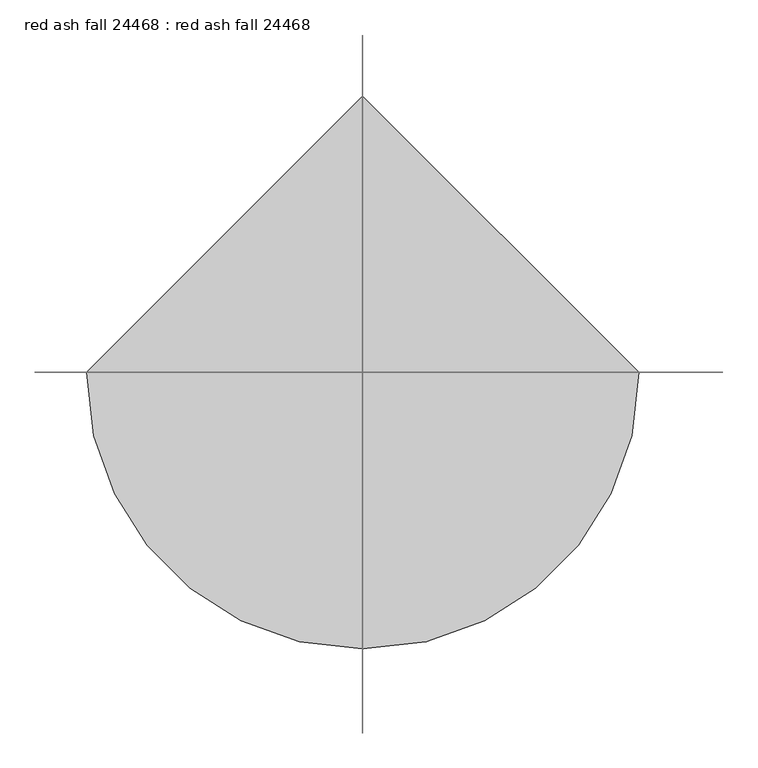
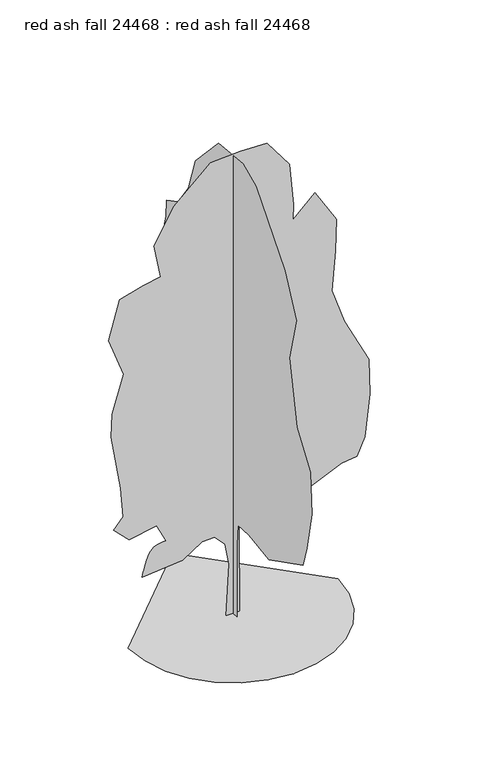
"""IFC4 building model written with IfcOpenShell, lengths in millimetres: proxy geometry, red ash fall 24468 : red ash fall 24468."""

from ifc_helpers import new_model, si_unit, origin, place, context, project, spatial, triangles, source, transform, mapped, element, save


def red_ash_fall_24468_red_ash_fall_24468_841d54ac(model_context):
    return source(origin(), model_context, "Body", "Tessellation", [
        triangles([(-1644.9506115, 0.0, 6.19e-05), (-1601.463295, -376.9127495, 6.19e-05), (-1477.6130058, -723.0483805, 6.19e-05), (-1283.3159992, -1028.488167, 6.19e-05), (-1028.488167, -1283.3159992, 6.19e-05), (-723.0483805, -1477.6130058, 6.19e-05), (-376.9127495, -1601.463295, 6.19e-05), (7.19e-05, -1644.9506115, 6.19e-05), (376.9127495, -1601.463295, 6.19e-05), (723.0483805, -1477.6130058, 6.19e-05), (1028.488167, -1283.3159992, 6.19e-05), (1283.3159992, -1028.488167, 6.19e-05), (1477.6130058, -723.0483805, 6.19e-05), (1601.463295, -376.9127495, 6.19e-05), (1644.9506115, 0.0001438, 6.19e-05), (-0.0002157, 1644.9506115, 6.19e-05), (-1.07e-05, -102.8462751, 0.0), (2.5e-05, -101.2465816, 1194.5531759), (3.23e-05, -129.8817524, 1537.8007565), (7e-07, -438.8252131, 1558.1640484), (-5.78e-05, -976.3902569, 1478.3064228), (-0.0001405, -1903.6900509, 1948.6758224), (-0.0001413, -2011.2029652, 2298.0931572), (-0.0001361, -2145.594326, 2943.1712242), (-0.0001119, -2105.2794903, 3615.1275925), (-5.81e-05, -1740.3808331, 4141.0085747), (-5.5e-06, -1527.397031, 5160.6396515), (-3.5e-06, -1715.5422329, 5886.3424484), (4.79e-05, -1406.4448208, 6531.4257477), (0.0001569, -626.9729948, 7458.7278671), (0.0001985, -273.1995851, 7618.189064), (0.0002662, 394.4006355, 7552.8093338), (0.0003121, 1026.0396246, 6880.8276764), (0.0003149, 1214.1899134, 6316.3894547), (0.0003323, 1496.4089516, 5913.2158081), (0.0003598, 1805.5114506, 5751.9512329), (0.0003531, 1818.9506012, 5483.1688019), (0.0003523, 1899.5853596, 5174.076622), (0.0003275, 1765.1941441, 4811.2124336), (0.0003297, 1886.146209, 4461.7849251), (0.0003279, 2007.0984192, 3977.9914902), (0.0003211, 1980.220118, 3843.6002747), (0.0002877, 1751.7549934, 3521.0461258), (0.0002729, 1737.3099449, 3077.5624397), (0.0002632, 1724.8766922, 2795.3433289), (0.0002542, 1738.3158428, 2445.9236687), (0.0002412, 1751.7549934, 1962.1149731), (0.0002172, 1563.6071754, 1814.2846069), (0.0001807, 1214.1899134, 1814.2846069), (0.0001827, 1375.4593575, 1317.0369061), (0.0001715, 1348.4948696, 1034.8838522), (0.0001516, 1103.0294746, 1227.8347927), (9.86e-05, 629.4621597, 1106.7073751), (9.8e-05, 551.7102922, 1357.0597538), (6.29e-05, 215.912475, 1354.0015102), (5.03e-05, 130.8009823, 1228.3325821), (3.27e-05, 79.5491688, 818.2830471), (1.17e-05, 112.1657825, 1.28e-05), (-110.8706308, 4.8e-06, 4.46e-05), (-66.7115076, -9.64e-05, 833.5001415), (-129.3072053, -0.000136, 1187.9415882), (-290.7865203, -0.00015, 1365.317244), (-483.63585, -0.0001408, 1358.6954098), (-796.2663677, -0.000103, 1155.7673893), (-1427.9079002, -6.9e-05, 1102.0109322), (-1419.1702068, -7.35e-05, 1136.7631714), (-1409.8433052, -7.82e-05, 1172.6914289), (-1399.343074, -8.32e-05, 1210.9717232), (-1387.0798691, -8.87e-05, 1252.7800724), (-1372.4647728, -9.49e-05, 1299.2874081), (-1354.9133732, -0.0001019, 1351.6722919), (-1333.8339912, -0.0001099, 1411.110815), (-1307.2681709, -0.0001176, 1466.2389908), (-1274.3547729, -0.0001239, 1506.5562973), (-1236.1533257, -0.0001289, 1534.5292992), (-1193.7200872, -0.0001329, 1552.6318279), (-1148.1144407, -0.0001362, 1563.327832), (-1100.3903915, -0.000139, 1569.0885269), (-1051.6097208, -0.0001415, 1572.3803318), (-1199.4401596, -0.0001703, 1868.0410641), (-1629.4947235, -0.0001418, 1787.4063057), (-1871.3989986, -0.0001601, 2029.3105808), (-1723.5686325, -0.0001874, 2204.0192482), (-1763.8834682, -0.0002433, 2687.8251823), (-1911.7164505, -0.0003442, 3588.2545235), (-1898.477869, -0.0003892, 3961.1515297), (-1719.9160938, -0.0004688, 4563.30867), (-1952.033757, -0.0005347, 5200.9494003), (-1777.3226189, -0.000616, 5819.1593399), (-1414.4661335, -0.0006447, 5926.6521973), (-1138.4116173, -0.0006626, 5975.3439926), (-1239.7574661, -0.0007228, 6517.9893585), (-930.6575832, -0.000802, 7068.9906097), (-352.7751603, -0.0008897, 7593.1190826), (117.5945209, -0.0009135, 7619.9924423), (534.2071818, -0.0009301, 7606.5560532), (883.6270237, -0.0008893, 7136.1737183), (947.8711401, -0.00081, 6447.504126), (938.6459038, -0.0007795, 6194.9520996), (1286.8008156, -0.0008333, 6517.9893585), (1622.7789997, -0.0007823, 5966.9875259), (1609.3398491, -0.0007196, 5446.5163879), (1549.4568764, -0.00064, 4800.6459274), (1743.7310646, -0.0005809, 4233.337532), (2131.7614494, -0.0005067, 3469.2048134), (2144.1338047, -0.0004386, 2892.8030777), (2066.2700981, -0.0003531, 2204.0192482), (1945.3180332, -0.0003141, 1921.7976665), (1703.4137581, -0.0003003, 1894.9193653), (1233.0443584, -0.0002542, 1679.8933914), (816.4288725, -0.0002007, 1384.2325138), (257.4769983, -0.0002049, 1624.5671173), (93.0507792, -0.0001766, 1447.6334404), (104.1551341, -4.6e-06, 3.52e-05)], [[15, 16, 1], [14, 15, 1], [14, 1, 2], [13, 14, 2], [13, 2, 3], [13, 3, 4], [12, 13, 4], [11, 12, 4], [11, 4, 5], [11, 5, 6], [11, 6, 7], [11, 7, 8], [11, 8, 9], [11, 9, 10], [50, 51, 52], [57, 58, 17], [57, 17, 18], [56, 57, 18], [56, 18, 19], [55, 56, 19], [49, 50, 52], [52, 53, 54], [49, 52, 54], [35, 36, 37], [46, 47, 48], [46, 48, 49], [21, 22, 23], [20, 21, 23], [20, 23, 24], [20, 24, 25], [20, 25, 26], [19, 20, 26], [19, 26, 27], [45, 46, 49], [31, 32, 33], [30, 31, 33], [29, 30, 33], [29, 33, 34], [28, 29, 34], [27, 28, 34], [19, 27, 34], [19, 34, 35], [19, 35, 37], [19, 37, 38], [19, 38, 39], [19, 39, 40], [19, 40, 41], [19, 41, 42], [19, 42, 43], [19, 43, 44], [19, 44, 45], [19, 45, 49], [19, 49, 54], [55, 19, 54], [64, 65, 66], [64, 66, 67], [64, 67, 68], [99, 100, 101], [64, 68, 69], [64, 69, 70], [64, 70, 71], [114, 59, 60], [113, 114, 60], [113, 60, 61], [113, 61, 62], [64, 71, 72], [64, 72, 73], [64, 73, 74], [64, 74, 75], [64, 75, 76], [64, 76, 77], [64, 77, 78], [64, 78, 79], [63, 64, 79], [81, 82, 83], [80, 81, 83], [99, 101, 102], [107, 108, 109], [110, 111, 112], [88, 89, 90], [87, 88, 90], [87, 90, 91], [80, 83, 84], [95, 96, 97], [95, 97, 98], [94, 95, 98], [93, 94, 98], [92, 93, 98], [91, 92, 98], [91, 98, 99], [87, 91, 99], [87, 99, 102], [87, 102, 103], [87, 103, 104], [86, 87, 104], [85, 86, 104], [84, 85, 104], [80, 84, 104], [80, 104, 105], [80, 105, 106], [80, 106, 107], [80, 107, 109], [80, 109, 110], [80, 110, 112], [79, 80, 112], [63, 79, 112], [62, 63, 112], [113, 62, 112]], closed=False),
    ])


if __name__ == "__main__":
    model = new_model("IFC4")
    model_context = context("Model", 3, world=origin())
    ifc_project = project(units=[si_unit("LENGTHUNIT", "METRE", prefix="MILLI")], contexts=[model_context])
    site = spatial("IfcSite", under=ifc_project)
    building = spatial("IfcBuilding", under=site)
    placement = place(None, origin())
    red_ash_fall_24468_red_ash_fall_24468_shape = red_ash_fall_24468_red_ash_fall_24468_841d54ac(model_context)
    element("IfcBuildingElementProxy", 1, Name="red ash fall 24468 : red ash fall 24468", ObjectType="red ash fall 24468 : red ash fall 24468", at=placement, inside=building, context=model_context, shape_type="MappedRepresentation", body=[
        mapped(red_ash_fall_24468_red_ash_fall_24468_shape, transform((0.0, 0.0, 0.0), x_axis=(1.0, 0.0, 0.0), y_axis=(0.0, 1.0, 0.0), z_axis=(0.0, 0.0, 1.0))),
    ])
    save(model, "model.ifc")

# Revit data of these elements
# Type "red ash fall 24468 : red ash fall 24468"
#   built-in parameter 1005195 = "RPC-16-G3AB-Q57X-UE54-U000-ST1L-LVER-AU"
#   Height = 0
